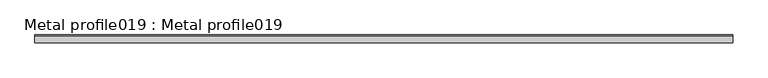
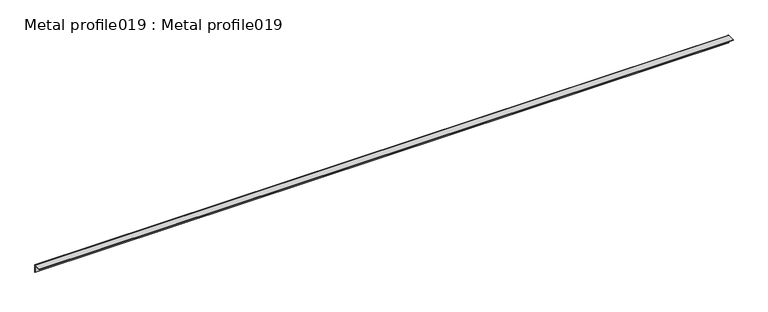
"""IFC4 building model written with IfcOpenShell, lengths in millimetres: proxy geometry, Metal profile019 : Metal profile019."""

from ifc_helpers import new_model, si_unit, point, frame, frame_2d, origin, place, context, project, spatial, polyline, circle_curve, trimmed, segment, composite_curve, outline, extrude, source, transform, mapped, element, save


def metal_profile019_metal_profile019_2dac266a(model_context):
    return source(origin(), model_context, "Body", "SweptSolid", [
        extrude(outline(composite_curve([segment(polyline([(-4505.9874811, 38426.4598437), (-4505.9874811, 38427.7398437), (-4485.0845714, 38427.7398437)]), True, "CONTINUOUS"), segment(trimmed(circle_curve(frame_2d((-4484.1942972, 38427.0998437)), 1.0964434), [point((-4485.0845714, 38427.7398437))], [point((-4483.5542972, 38426.2095695))], False, "CARTESIAN"), True, "CONTINUOUS"), segment(polyline([(-4483.5542972, 38426.2095695), (-4483.5542972, 38405.3066598), (-4484.8342972, 38405.3066598), (-4484.8342972, 38426.4598437), (-4505.9874811, 38426.4598437)]), True, "CONTINUOUS")], self_intersect=False)), frame((12383.0178845, 0.0, 0.0), z_axis=(1.0, 0.0, 0.0), x_axis=(0.0, 1.0, 0.0)), (0.0, 0.0, 1.0), 2000.0),
    ])


if __name__ == "__main__":
    model = new_model("IFC4")
    model_context = context("Model", 3, world=origin())
    ifc_project = project(units=[si_unit("LENGTHUNIT", "METRE", prefix="MILLI")], contexts=[model_context])
    site = spatial("IfcSite", under=ifc_project)
    building = spatial("IfcBuilding", under=site)
    placement = place(None, origin())
    metal_profile019_metal_profile019_shape = metal_profile019_metal_profile019_2dac266a(model_context)
    element("IfcBuildingElementProxy", 1, Name="Metal profile019 : Metal profile019", ObjectType="Metal profile019 : Metal profile019", at=placement, inside=building, context=model_context, shape_type="MappedRepresentation", body=[
        mapped(metal_profile019_metal_profile019_shape, transform((0.0, 0.0, 0.0), x_axis=(1.0, 0.0, 0.0), y_axis=(0.0, 1.0, 0.0), z_axis=(0.0, 0.0, 1.0))),
    ])
    save(model, "model.ifc")

# Revit data of these elements
# Type "Metal profile019 : Metal profile019"
#   NameOverride = "Metal profile019"
# Element 1 (IfcBuildingElementProxy, "Metal profile019 : Metal profile019")
#   Materials on its faces: "CORNER BEAD"
# Materials
#   "CORNER BEAD": class "Unassigned", colour RGB 253 236 176, transparency 0, Cost = 0
